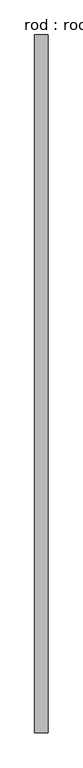
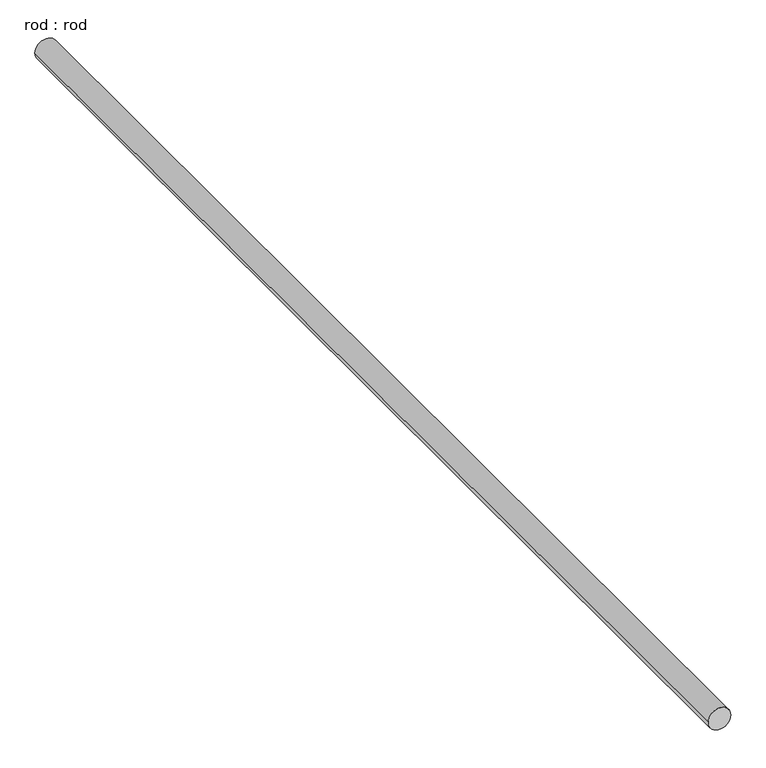
"""IFC4 building model written with IfcOpenShell, lengths in millimetres: proxy geometry, rod : rod."""

from ifc_helpers import new_model, si_unit, point, frame, frame_2d, origin, place, context, project, spatial, circle_curve, trimmed, segment, composite_curve, outline, extrude, source, transform, mapped, element, save


def rod_rod_0aac5bb3(model_context):
    return source(origin(), model_context, "Body", "SweptSolid", [
        extrude(outline(composite_curve([segment(trimmed(circle_curve(frame_2d((0.0108462, 0.0)), 200.0), [point((0.0108462, 200.0))], [point((0.0108462, -200.0))], False, "CARTESIAN"), True, "CONTINUOUS"), segment(trimmed(circle_curve(frame_2d((0.0108462, 0.0)), 200.0), [point((0.0108462, -200.0))], [point((0.0108462, 200.0))], False, "CARTESIAN"), True, "CONTINUOUS")], self_intersect=False)), frame((0.0, -6206.3785275, 0.0), z_axis=(0.0, 1.0, 0.0), x_axis=(0.0, 0.0, 1.0)), (0.0, 0.0, 1.0), 20598.2142857),
    ])


if __name__ == "__main__":
    model = new_model("IFC4")
    model_context = context("Model", 3, world=origin())
    ifc_project = project(units=[si_unit("LENGTHUNIT", "METRE", prefix="MILLI")], contexts=[model_context])
    site = spatial("IfcSite", under=ifc_project)
    building = spatial("IfcBuilding", under=site)
    placement = place(None, origin())
    rod_rod_shape = rod_rod_0aac5bb3(model_context)
    element("IfcBuildingElementProxy", 1, Name="rod : rod", ObjectType="rod : rod", at=placement, inside=building, context=model_context, shape_type="MappedRepresentation", body=[
        mapped(rod_rod_shape, transform((0.0, 0.0, 0.0), x_axis=(1.0, 0.0, 0.0), y_axis=(0.0, 1.0, 0.0), z_axis=(0.0, 0.0, 1.0))),
    ])
    save(model, "model.ifc")

# Revit data of these elements
# Type "rod : rod"
#   Default Elevation = 0
